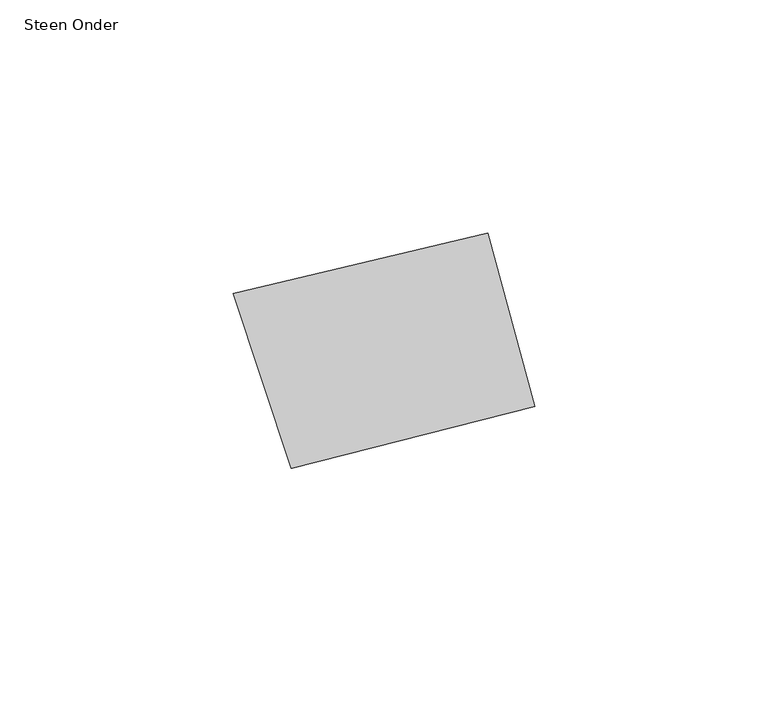
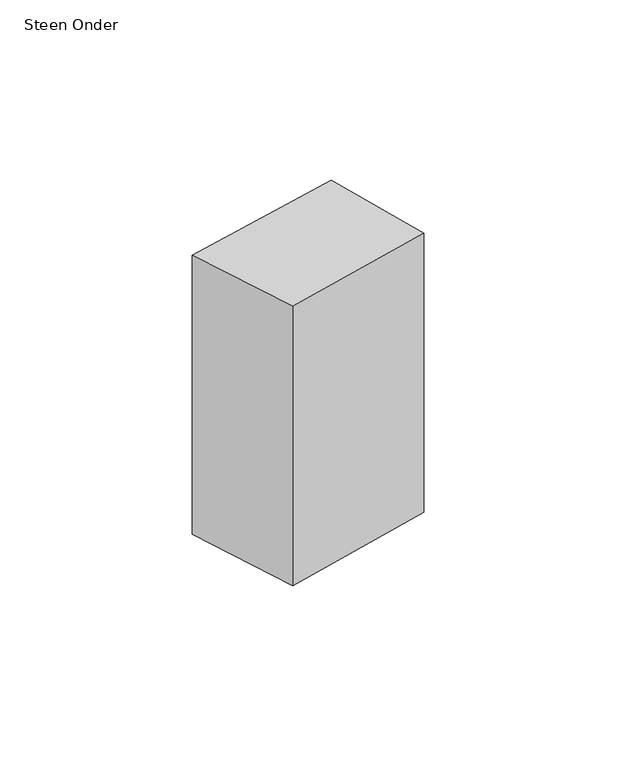
"""IFC4 building model written with IfcOpenShell, lengths in millimetres: proxy geometry, 00_GMA_steen_versie_4 : Steen Onder."""

from ifc_helpers import new_model, si_unit, origin, origin_with_axes, place, context, project, spatial, polyline, outline, extrude, source, transform, mapped, element, save


def steen_onder_14dc429e(model_context):
    return source(origin(), model_context, "Body", "SweptSolid", [
        extrude(outline(polyline([(96.3163118, 83.6914244), (106.2982906, 46.6153559), (54.2309113, 33.3308832), (41.8319917, 70.7418151), (96.3163118, 83.6914244)])), origin_with_axes(), (0.0, 0.0, 1.0), 100.0),
    ])


if __name__ == "__main__":
    model = new_model("IFC4")
    model_context = context("Model", 3, world=origin())
    ifc_project = project(units=[si_unit("LENGTHUNIT", "METRE", prefix="MILLI")], contexts=[model_context])
    site = spatial("IfcSite", under=ifc_project)
    building = spatial("IfcBuilding", under=site)
    placement = place(None, origin())
    steen_onder_shape = steen_onder_14dc429e(model_context)
    element("IfcBuildingElementProxy", 1, Name="00_GMA_steen_versie_4 : Steen Onder", ObjectType="00_GMA_steen_versie_4 : Steen Onder", at=placement, inside=building, context=model_context, shape_type="MappedRepresentation", body=[
        mapped(steen_onder_shape, transform((0.0, 0.0, 0.0), x_axis=(1.0, 0.0, 0.0), y_axis=(0.0, 1.0, 0.0), z_axis=(0.0, 0.0, 1.0))),
    ])
    save(model, "model.ifc")

# Revit data of these elements
# Type "00_GMA_steen_versie_4 : Steen Onder"
#   StootVoegHalfBoven [instance default] = 5 mm
#   StootVoegHalf [instance default] = 5 mm
#   StootVoegBreedteOnder = 10 mm
#   StootVoegBreedteBoven = 10 mm
#   Steendikte = 100 mm
#   LintVoegOnderHalf = 0 mm
#   LintVoegOnder = 0 mm
#   LintVoegBovenHalf = 5 mm
#   LintVoegBoven = 10 mm
#   materiaal = none
#   MateriaalVoeg = none
#   Default Elevation = 0
